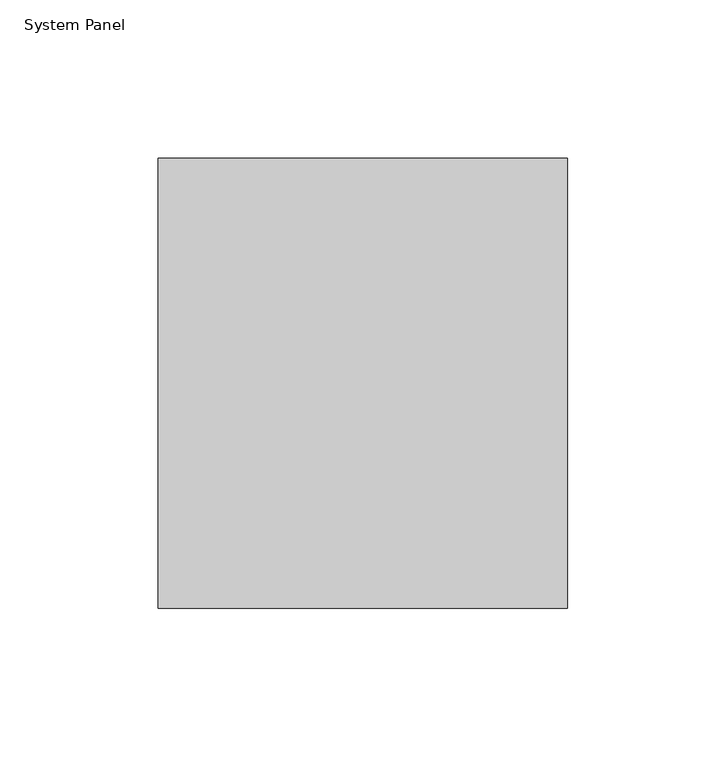
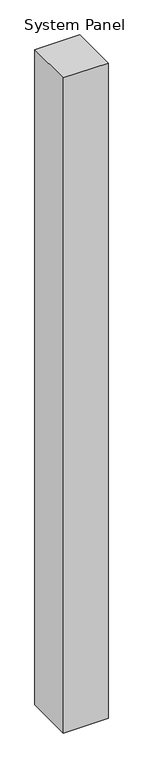
"""IFC4 building model written with IfcOpenShell, lengths in millimetres: plate geometry, System Panel : NLRS_21_CWP_hsb-vulling minerale wol 142 _gen_rsf."""

import ifcopenshell
import ifcopenshell.guid

model = None  # the IFC model being written
_history = None  # IfcOwnerHistory: only IFC2X3 demands one
_inside = {}  # id of a spatial element -> (the spatial element, [elements in it])
_under = {}  # id of a project, library or spatial element -> (it, [spatial elements below it])
_declared = {}  # id of a project -> (the project, [libraries it declares])
_typed = {}  # id of a type object -> (the type object, [elements of that type])
_made_of = {}  # id of a material, layer set ... -> (it, [elements and type objects made of it])


def new_model(schema):
    """Start an empty IFC model of exactly this schema.

    Asked for "IFC4X3", IfcOpenShell would pick the latest addendum, in which some entities
    have other attributes; the version numbers below select the first issue.
    IFC2X3 requires an IfcOwnerHistory on every rooted entity: one is made here for all.
    """
    global model, _history
    if schema == "IFC4X3":
        model = ifcopenshell.file(schema_version=(4, 3, 0, 0))
    else:
        model = ifcopenshell.file(schema=schema)
    _inside.clear()
    _under.clear()
    _declared.clear()
    _typed.clear()
    _made_of.clear()
    _history = None
    if model.schema == "IFC2X3":
        org = make("IfcOrganization", Name="unknown")
        user = make(
            "IfcPersonAndOrganization",
            ThePerson=make("IfcPerson", FamilyName="unknown"),
            TheOrganization=org,
        )
        app = make(
            "IfcApplication",
            ApplicationDeveloper=org,
            Version="unknown",
            ApplicationFullName="unknown",
            ApplicationIdentifier="unknown",
        )
        _history = make(
            "IfcOwnerHistory",
            OwningUser=user,
            OwningApplication=app,
            ChangeAction="ADDED",
            CreationDate=0,
        )
    return model


def make(cls, **values):
    """One entity of the class cls with the attributes given. An attribute that is None is left unset."""
    return model.create_entity(
        cls, **{name: value for name, value in values.items() if value is not None}
    )


def rooted(cls, **values):
    """An entity with a GlobalId (a new one), such as an element, a storey or a relation."""
    return make(cls, GlobalId=ifcopenshell.guid.new(), OwnerHistory=_history, **values)


def si_unit(unit_type, name, prefix=None):
    """IfcSIUnit, for example si_unit("LENGTHUNIT", "METRE", prefix="MILLI")."""
    return make("IfcSIUnit", UnitType=unit_type, Prefix=prefix, Name=name)


def assignment(units):
    """IfcUnitAssignment: the units of a project."""
    return None if units is None else make("IfcUnitAssignment", Units=units)


def point(xyz):
    """IfcCartesianPoint."""
    return None if xyz is None else make("IfcCartesianPoint", Coordinates=xyz)


def direction(xyz):
    """IfcDirection."""
    return None if xyz is None else make("IfcDirection", DirectionRatios=xyz)


def frame(location, z_axis=None, x_axis=None):
    """IfcAxis2Placement3D, a coordinate frame: its origin and axes. An axis left out is left unset."""
    return make(
        "IfcAxis2Placement3D",
        Location=point(location),
        Axis=direction(z_axis),
        RefDirection=direction(x_axis),
    )


def origin():
    """The frame at (0, 0, 0) with its axes left unset."""
    return frame((0.0, 0.0, 0.0))


def origin_with_axes():
    """The frame at (0, 0, 0) with the z axis (0, 0, 1) and the x axis (1, 0, 0) written out."""
    return frame((0.0, 0.0, 0.0), z_axis=(0.0, 0.0, 1.0), x_axis=(1.0, 0.0, 0.0))


def place(relative_to, where):
    """IfcLocalPlacement: puts the frame where relative to a parent placement (None: the world)."""
    return make(
        "IfcLocalPlacement", PlacementRelTo=relative_to, RelativePlacement=where
    )


def context(
    kind, dimensions, precision=None, world=None, true_north=None, identifier=None
):
    """IfcGeometricRepresentationContext, for example the 3D "Model" context."""
    return make(
        "IfcGeometricRepresentationContext",
        ContextIdentifier=identifier,
        ContextType=kind,
        CoordinateSpaceDimension=dimensions,
        Precision=precision,
        WorldCoordinateSystem=world,
        TrueNorth=true_north,
    )


def project(units=None, contexts=None):
    """IfcProject with its units and contexts."""
    return rooted(
        "IfcProject",
        Name="project",
        RepresentationContexts=contexts,
        UnitsInContext=assignment(units),
    )


def spatial(cls, under=None, at=None, **own):
    """A site, building, storey or space (cls), placed at a placement, below another one or the project."""
    s = rooted(cls, ObjectPlacement=at, **own)
    if under is not None:
        _under.setdefault(under.id(), (under, []))[1].append(s)
    return s


def polyline(points):
    """IfcPolyline through the points."""
    return make("IfcPolyline", Points=[point(p) for p in points])


def outline(outer, holes=None, kind="AREA"):
    """IfcArbitraryClosedProfileDef: a profile drawn as a closed curve; with holes, ...WithVoids."""
    if holes is None:
        return make("IfcArbitraryClosedProfileDef", ProfileType=kind, OuterCurve=outer)
    return make(
        "IfcArbitraryProfileDefWithVoids",
        ProfileType=kind,
        OuterCurve=outer,
        InnerCurves=holes,
    )


def extrude(swept, where, along, depth):
    """IfcExtrudedAreaSolid: the profile swept, set in the frame where, extruded along a direction by depth."""
    return make(
        "IfcExtrudedAreaSolid",
        SweptArea=swept,
        Position=where,
        ExtrudedDirection=direction(along),
        Depth=depth,
    )


def shape(context_of_items, identifier, shape_type, items):
    """IfcShapeRepresentation: the items that make up one representation, for example the "Body"."""
    return make(
        "IfcShapeRepresentation",
        ContextOfItems=context_of_items,
        RepresentationIdentifier=identifier,
        RepresentationType=shape_type,
        Items=items,
    )


def source(mapping_origin, context_of_items, identifier, shape_type, items):
    """IfcRepresentationMap: a shape defined once, which mapped items show again and again."""
    return make(
        "IfcRepresentationMap",
        MappingOrigin=mapping_origin,
        MappedRepresentation=shape(context_of_items, identifier, shape_type, items),
    )


def transform(
    local_origin,
    x_axis=None,
    y_axis=None,
    z_axis=None,
    scale=None,
    scale2=None,
    scale3=None,
    uniform=True,
):
    """IfcCartesianTransformationOperator3D, or its non-uniform kind. x_axis, y_axis, z_axis: its Axis1, 2, 3."""
    if uniform:
        return make(
            "IfcCartesianTransformationOperator3D",
            Axis1=direction(x_axis),
            Axis2=direction(y_axis),
            LocalOrigin=point(local_origin),
            Scale=scale,
            Axis3=direction(z_axis),
        )
    return make(
        "IfcCartesianTransformationOperator3DnonUniform",
        Axis1=direction(x_axis),
        Axis2=direction(y_axis),
        LocalOrigin=point(local_origin),
        Scale=scale,
        Axis3=direction(z_axis),
        Scale2=scale2,
        Scale3=scale3,
    )


def mapped(mapping_source, mapping_target):
    """IfcMappedItem: shows the shape of a source again, moved by a transform."""
    return make(
        "IfcMappedItem", MappingSource=mapping_source, MappingTarget=mapping_target
    )


def made_of(thing, what):
    """Note that an element or type object is made of a material, layer set ...; save() writes the relation."""
    if what is not None:
        _made_of.setdefault(what.id(), (what, []))[1].append(thing)
    return thing


def element(
    cls,
    number,
    at=None,
    inside=None,
    cuts=None,
    type_object=None,
    material=None,
    context=None,
    identifier="Body",
    shape_type=None,
    held_by="IfcProductDefinitionShape",
    body=None,
    shapes=None,
    **own,
):
    """One element of the class cls, such as IfcWall. Its Tag is "e" and its number.

    at: its placement. inside: the storey or other place that contains it. cuts: it is an
    opening in that element (IfcRelVoidsElement). A single representation is given by context,
    identifier, shape_type and body (its items); several are given by shapes. held_by: the class
    of the entity that holds the representations. save() writes the other relations.
    """
    e = rooted(cls, Tag="e%d" % number, ObjectPlacement=at, **own)
    if body is not None:
        shapes = [shape(context, identifier, shape_type, body)]
    if shapes is not None:
        e.Representation = make(held_by, Representations=shapes)
    if inside is not None:
        _inside.setdefault(inside.id(), (inside, []))[1].append(e)
    if cuts is not None:
        rooted(
            "IfcRelVoidsElement", RelatingBuildingElement=cuts, RelatedOpeningElement=e
        )
    if type_object is not None:
        _typed.setdefault(type_object.id(), (type_object, []))[1].append(e)
    return made_of(e, material)


def aggregate(whole, parts):
    """IfcRelAggregates: a whole, such as a stair, and the parts it consists of."""
    return rooted("IfcRelAggregates", RelatingObject=whole, RelatedObjects=parts)


def save(model, path):
    """Write the relations noted so far, then the file.

    IfcRelAggregates (storeys below a building ...), IfcRelContainedInSpatialStructure (elements
    in a storey), IfcRelDefinesByType, IfcRelAssociatesMaterial and IfcRelDeclares: one each for
    every whole, place, type object, material and project.
    """
    for whole, parts in _under.values():
        aggregate(whole, parts)
    for where, things in _inside.values():
        rooted(
            "IfcRelContainedInSpatialStructure",
            RelatedElements=things,
            RelatingStructure=where,
        )
    for kind, things in _typed.values():
        rooted("IfcRelDefinesByType", RelatedObjects=things, RelatingType=kind)
    for what, things in _made_of.values():
        rooted("IfcRelAssociatesMaterial", RelatedObjects=things, RelatingMaterial=what)
    for by, libraries in _declared.values():
        rooted("IfcRelDeclares", RelatingContext=by, RelatedDefinitions=libraries)
    model.write(path)


def system_panel_6860f7c2(model_context):
    return source(origin(), model_context, "Body", "SweptSolid", [
        extrude(outline(polyline([(64.577947, -71.0), (-64.577947, -71.0), (-64.577947, 71.0), (64.577947, 71.0), (64.577947, -71.0)])), origin_with_axes(), (0.0, 0.0, 1.0), 2000.0),
    ])


if __name__ == "__main__":
    model = new_model("IFC4")
    model_context = context("Model", 3, world=origin())
    ifc_project = project(units=[si_unit("LENGTHUNIT", "METRE", prefix="MILLI")], contexts=[model_context])
    site = spatial("IfcSite", under=ifc_project)
    building = spatial("IfcBuilding", under=site)
    placement = place(None, origin())
    system_panel_shape = system_panel_6860f7c2(model_context)
    element("IfcPlate", 1, ObjectType="System Panel : NLRS_21_CWP_hsb-vulling minerale wol 142 _gen_rsf", at=placement, inside=building, context=model_context, shape_type="MappedRepresentation", body=[
        mapped(system_panel_shape, transform((0.0, 0.0, 0.0), x_axis=(1.0, 0.0, 0.0), y_axis=(0.0, 1.0, 0.0), z_axis=(0.0, 0.0, 1.0))),
    ])
    save(model, "model.ifc")

# Revit data of these elements
# Type "System Panel : NLRS_21_CWP_hsb-vulling minerale wol 142 _gen_rsf"
#   Export Type to IFC As = "IfcWall"
#   Type IfcGUID = "07M7mRoiH1CR8m_RSKIwpC"
#   Assembly Code = "21.23"
# Element 1 (IfcPlate, "System Panel : NLRS_21_CWP_hsb-vulling minerale wol 142 _gen_rsf")
#   Materials on its faces: "NLRS_m1_isolatie minerale wol_gen_rsf"
# Materials
#   "NLRS_m1_isolatie minerale wol_gen_rsf": class "M - Anorganische materialen", colour RGB 200 200 140, transparency 0, Keynote = "m1", Manufacturer = "Revit Standards Foundation", URL = "www.revitstandards.org", Description = "isolatie minerale wol", Cost = 0
